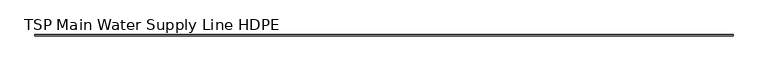
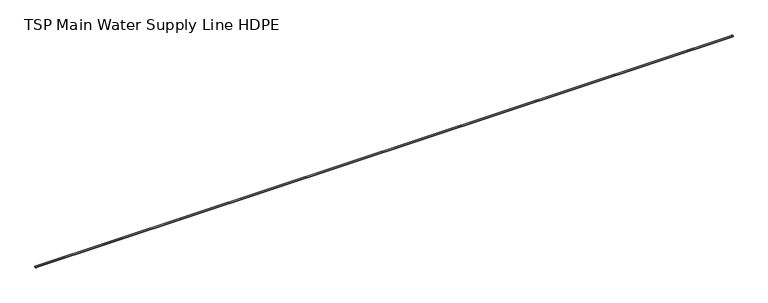
"""IFC4 building model written with IfcOpenShell, lengths in millimetres: flow terminal geometry, TSP Main Water Supply Line HDPE : HDPE Fresh Water Supply."""

from ifc_helpers import new_model, si_unit, point, frame, origin, origin_2d, place, context, project, spatial, circle_curve, trimmed, segment, composite_curve, outline, extrude, source, transform, mapped, element, save


def tsp_main_water_supply_line_hdpe_cb4fbaf4(model_context):
    return source(origin(), model_context, "Body", "SweptSolid", [
        extrude(outline(composite_curve([segment(trimmed(circle_curve(origin_2d(), 16.0), [point((-16.0, 0.0))], [point((16.0, 0.0))], False, "CARTESIAN"), True, "CONTINUOUS"), segment(trimmed(circle_curve(origin_2d(), 16.0), [point((16.0, 0.0))], [point((-16.0, 0.0))], False, "CARTESIAN"), True, "CONTINUOUS")], self_intersect=False), holes=[composite_curve([segment(trimmed(circle_curve(origin_2d(), 15.0), [point((-15.0, 0.0))], [point((15.0, 0.0))], True, "CARTESIAN"), True, "CONTINUOUS"), segment(trimmed(circle_curve(origin_2d(), 15.0), [point((15.0, 0.0))], [point((-15.0, 0.0))], True, "CARTESIAN"), True, "CONTINUOUS")], self_intersect=False)]), frame((0.0, 0.0, 0.0), z_axis=(1.0, 0.0, 0.0), x_axis=(0.0, 1.0, 0.0)), (0.0, 0.0, 1.0), 15746.0266191),
    ])


if __name__ == "__main__":
    model = new_model("IFC4")
    model_context = context("Model", 3, world=origin())
    ifc_project = project(units=[si_unit("LENGTHUNIT", "METRE", prefix="MILLI")], contexts=[model_context])
    site = spatial("IfcSite", under=ifc_project)
    building = spatial("IfcBuilding", under=site)
    placement = place(None, origin())
    tsp_main_water_supply_line_hdpe_shape = tsp_main_water_supply_line_hdpe_cb4fbaf4(model_context)
    element("IfcFlowTerminal", 1, ObjectType="TSP Main Water Supply Line HDPE : HDPE Fresh Water Supply", at=placement, inside=building, context=model_context, shape_type="MappedRepresentation", body=[
        mapped(tsp_main_water_supply_line_hdpe_shape, transform((0.0, 0.0, 0.0), x_axis=(1.0, 0.0, 0.0), y_axis=(0.0, 1.0, 0.0), z_axis=(0.0, 0.0, 1.0))),
    ])
    save(model, "model.ifc")

# Revit data of these elements
# Type "TSP Main Water Supply Line HDPE : HDPE Fresh Water Supply"
#   Model = "TSP_110SFWSP"
#   Pipe length [instance default] = 1200 mm
#   Pipe dia = 30 mm
#   built-in parameter 1001306 [instance default] = 3.93701 (stored number, unit not read)
#   Default Elevation = 0
# Element 1 (IfcFlowTerminal, "TSP Main Water Supply Line HDPE : HDPE Fresh Water Supply")
#   Pipe length = 15746.027 mm
#   built-in parameter 1001306 = 51.6602 (stored number, unit not read)
#   Materials on its faces: "Aluminum, Anodized Blue"
# Materials
#   "Aluminum, Anodized Blue": class "Metal", colour RGB 120 120 120, transparency 0, Description = "Anodized aluminum, blue", Cost = 0
